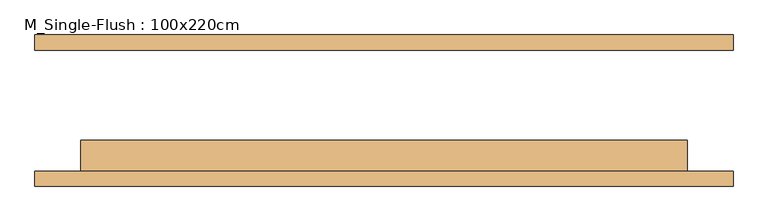
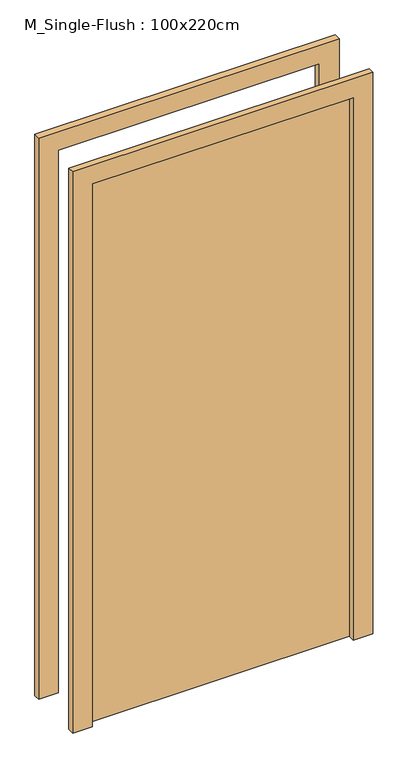
"""IFC4 building model written with IfcOpenShell, lengths in millimetres: door geometry, M_Single-Flush : 100x220cm."""

from ifc_helpers import new_model, si_unit, frame, origin, origin_with_axes, place, context, project, spatial, polyline, outline, extrude, source, transform, mapped, element, save


def m_single_flush_100x220cm_6cbb3975(model_context):
    return source(origin(), model_context, "Body", "SweptSolid", [
        extrude(outline(polyline([(2276.0, -576.0), (0.0, -576.0), (0.0, -500.0), (2200.0, -500.0), (2200.0, 500.0), (0.0, 500.0), (0.0, 576.0), (2276.0, 576.0), (2276.0, -576.0)])), frame((0.0, -125.0, 0.0), z_axis=(0.0, 1.0, 0.0), x_axis=(0.0, 0.0, 1.0)), (0.0, 0.0, 1.0), 25.0),
        extrude(outline(polyline([(2276.0, 576.0), (2276.0, -576.0), (0.0, -576.0), (0.0, -500.0), (2200.0, -500.0), (2200.0, 500.0), (0.0, 500.0), (0.0, 576.0), (2276.0, 576.0)])), frame((0.0, 100.0, 0.0), z_axis=(0.0, 1.0, 0.0), x_axis=(0.0, 0.0, 1.0)), (0.0, 0.0, 1.0), 25.0),
        extrude(outline(polyline([(500.0, -49.0), (500.0, -100.0), (-500.0, -100.0), (-500.0, -49.0), (500.0, -49.0)])), origin_with_axes(), (0.0, 0.0, 1.0), 2200.0),
    ])


if __name__ == "__main__":
    model = new_model("IFC4")
    model_context = context("Model", 3, world=origin())
    ifc_project = project(units=[si_unit("LENGTHUNIT", "METRE", prefix="MILLI")], contexts=[model_context])
    site = spatial("IfcSite", under=ifc_project)
    building = spatial("IfcBuilding", under=site)
    placement = place(None, origin())
    m_single_flush_100x220cm_shape = m_single_flush_100x220cm_6cbb3975(model_context)
    element("IfcDoor", 1, ObjectType="M_Single-Flush : 100x220cm", at=placement, inside=building, context=model_context, shape_type="MappedRepresentation", body=[
        mapped(m_single_flush_100x220cm_shape, transform((0.0, 0.0, 0.0), x_axis=(1.0, 0.0, 0.0), y_axis=(0.0, 1.0, 0.0), z_axis=(0.0, 0.0, 1.0))),
    ])
    save(model, "model.ifc")

# Revit data of these elements
# Type "M_Single-Flush : 100x220cm"
#   Type Mark = "44"
#   Construction Type Id = "MDOOR"
#   Analytic Construction = "Metal"
#   Thickness = 5.10 cm
#   Heat Transfer Coefficient (U) = 3.7021 W/(m²·K)
#   Height = 220.00 cm
#   Trim Projection Ext = 2.50 cm
#   Trim Projection Int = 2.50 cm
#   Trim Width = 7.60 cm
#   Width = 100.00 cm
#   Define Thermal Properties by = 1
#   Door Material = Door - Panel
#   Frame Material = Door - Frame
#   Visual Light Transmittance = 0
#   Solar Heat Gain Coefficient = 0
#   Function = (empty or 0)
#   Wall Closure = (empty or 0)
# Element 1 (IfcDoor, "M_Single-Flush : 100x220cm")
#   Materials on its faces: "Door - Frame", "Door - Panel"
# Materials
#   "Door - Panel": class "Wood", colour RGB 210 159 95, transparency 0, Cost = 0
#   "Door - Frame": class "Miscellaneous", colour RGB 118 70 51, transparency 0, Cost = 0
